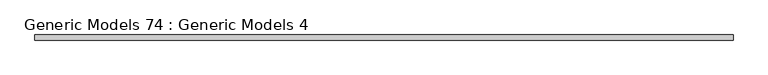
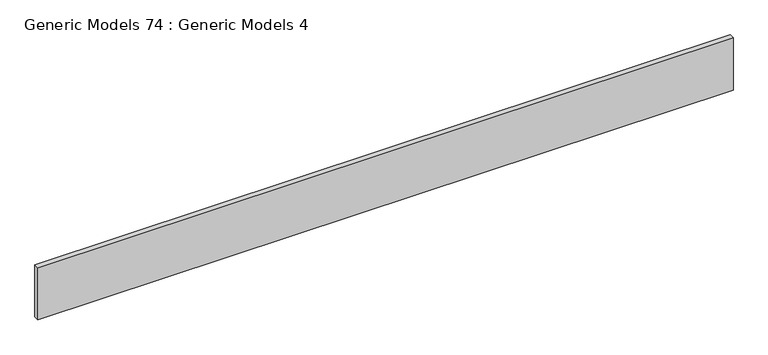
"""IFC4 building model written with IfcOpenShell, lengths in millimetres: proxy geometry, Generic Models 74 : Generic Models 4."""

from ifc_helpers import new_model, si_unit, frame, origin, place, context, project, spatial, polyline, outline, extrude, source, transform, mapped, element, save


def generic_models_74_generic_models_4_ad37d0a4(model_context):
    return source(origin(), model_context, "Body", "SweptSolid", [
        extrude(outline(polyline([(24896.3074258, -8057.0818256), (24896.3074258, -8069.7818256), (23155.3573109, -8069.7818256), (23155.3573109, -8057.0818256), (24896.3074258, -8057.0818256)])), frame((0.0, 0.0, 123145.296), z_axis=(0.0, 0.0, 1.0), x_axis=(1.0, 0.0, 0.0)), (0.0, 0.0, 1.0), 138.3422763),
    ])


if __name__ == "__main__":
    model = new_model("IFC4")
    model_context = context("Model", 3, world=origin())
    ifc_project = project(units=[si_unit("LENGTHUNIT", "METRE", prefix="MILLI")], contexts=[model_context])
    site = spatial("IfcSite", under=ifc_project)
    building = spatial("IfcBuilding", under=site)
    placement = place(None, origin())
    generic_models_74_generic_models_4_shape = generic_models_74_generic_models_4_ad37d0a4(model_context)
    element("IfcBuildingElementProxy", 1, Name="Generic Models 74 : Generic Models 4", ObjectType="Generic Models 74 : Generic Models 4", at=placement, inside=building, context=model_context, shape_type="MappedRepresentation", body=[
        mapped(generic_models_74_generic_models_4_shape, transform((0.0, 0.0, 0.0), x_axis=(1.0, 0.0, 0.0), y_axis=(0.0, 1.0, 0.0), z_axis=(0.0, 0.0, 1.0))),
    ])
    save(model, "model.ifc")

# Revit data of these elements
# Element 1 (IfcBuildingElementProxy, "Generic Models 74 : Generic Models 4")
#   Materials on its faces: "_CONCRETE EXPANSION JOINT - MINERAL FIBER"
# Materials
#   "_CONCRETE EXPANSION JOINT - MINERAL FIBER": class "Generic", colour RGB 190 220 196, transparency 0, Cost = 0
